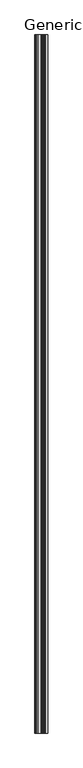
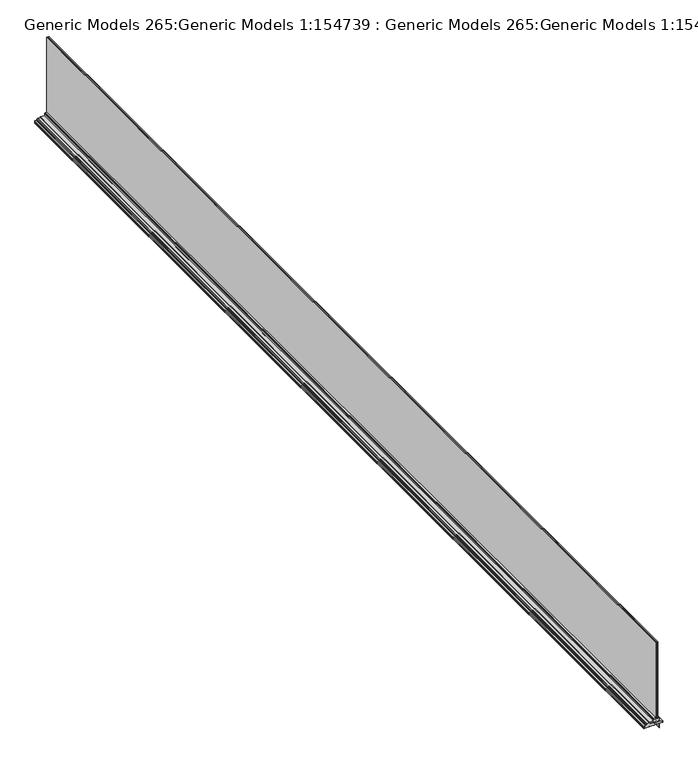
"""IFC4 building model written with IfcOpenShell, lengths in millimetres: proxy geometry, Generic Models 265:Generic Models 1:154739 : Generic Models 265:Generic Models 1:154739."""

from ifc_helpers import new_model, si_unit, point, frame, frame_2d, origin, place, context, project, spatial, polyline, circle_curve, trimmed, segment, composite_curve, outline, extrude, source, transform, mapped, element, save


def generic_models_265_generic_models_1_154739_generic_models_7b3244d4(model_context):
    return source(origin(), model_context, "Body", "SweptSolid", [
        extrude(outline(polyline([(1586.584463, 8383.5218843), (1586.584463, 496.8218843), (1581.821963, 496.8218843), (1581.821963, 8383.5218843), (1586.584463, 8383.5218843)])), frame((0.0, 0.0, 228.0707428), z_axis=(0.0, 0.0, 1.0), x_axis=(1.0, 0.0, 0.0)), (0.0, 0.0, 1.0), 602.3375481),
        extrude(outline(polyline([(1581.028213, 8383.5218843), (1581.028213, 496.8218843), (1574.679131, 496.8218843), (1574.679131, 8383.5218843), (1581.028213, 8383.5218843)])), frame((0.0, 0.0, 228.0707428), z_axis=(0.0, 0.0, 1.0), x_axis=(1.0, 0.0, 0.0)), (0.0, 0.0, 1.0), 6.35),
        extrude(outline(polyline([(1573.885381, 8383.5218843), (1573.885381, 496.8218843), (1569.122881, 496.8218843), (1569.122881, 8383.5218843), (1573.885381, 8383.5218843)])), frame((0.0, 0.0, 228.0707428), z_axis=(0.0, 0.0, 1.0), x_axis=(1.0, 0.0, 0.0)), (0.0, 0.0, 1.0), 602.3375481),
        extrude(outline(composite_curve([segment(polyline([(236.1161928, 1588.4013551), (231.8807536, 1588.4013551), (230.8576116, 1587.378213), (227.2769928, 1587.378213), (227.2769928, 1565.9408422), (229.6652816, 1568.329131), (239.5966816, 1568.329131), (238.5840316, 1556.5014505), (236.4216816, 1556.5014505), (236.4216816, 1552.733531), (228.8778816, 1552.733531), (228.8778816, 1554.333731), (227.2769928, 1554.333731), (227.2769928, 1552.453213), (208.9889928, 1552.453213)]), True, "CONTINUOUS"), segment(trimmed(circle_curve(frame_2d((208.9889928, 1553.266013)), 0.8128), [point((208.9889928, 1552.453213))], [point((208.1761928, 1553.266013))], False, "CARTESIAN"), True, "CONTINUOUS"), segment(polyline([(208.1761928, 1553.266013), (208.1761928, 1566.601013)]), True, "CONTINUOUS"), segment(trimmed(circle_curve(frame_2d((208.1761928, 1568.582213)), 1.9812), [point((208.1761928, 1566.601013))], [point((208.1761928, 1570.563413))], True, "CARTESIAN"), True, "CONTINUOUS"), segment(polyline([(208.1761928, 1570.563413), (208.1761928, 1582.755413), (202.8675928, 1582.755413), (202.8675928, 1588.368813), (210.7923928, 1588.368813), (210.7923928, 1590.273813), (207.4903928, 1590.273813), (207.4903928, 1591.950213), (205.4583928, 1591.950213), (205.4583928, 1594.515613)]), True, "CONTINUOUS"), segment(trimmed(circle_curve(frame_2d((207.8459928, 1594.515613)), 2.3876), [point((205.4583928, 1594.515613))], [point((207.8459928, 1596.903213))], False, "CARTESIAN"), True, "CONTINUOUS"), segment(polyline([(207.8459928, 1596.903213), (230.1471928, 1596.903213), (230.1471928, 1594.515613), (237.9530163, 1591.9802525), (238.1425666, 1589.537213), (236.1161928, 1589.537213), (236.1161928, 1588.4013551)]), True, "CONTINUOUS")], self_intersect=False)), frame((0.0, 496.8218843, 0.0), z_axis=(0.0, 1.0, 0.0), x_axis=(0.0, 0.0, 1.0)), (0.0, 0.0, 1.0), 7886.7),
        extrude(outline(composite_curve([segment(polyline([(190.97406, 1480.6982627), (183.0238428, 1480.6982627), (183.0238428, 1498.7668061), (186.1988428, 1498.7668061), (186.1988428, 1501.05281), (183.0238428, 1501.05281), (183.0238428, 1518.5605591), (186.1988428, 1518.5605591), (186.1988428, 1520.846563), (183.0238428, 1520.846563), (183.0238428, 1537.8736627), (185.1066428, 1537.8736627), (185.1066428, 1541.0486627), (183.0238428, 1541.0486627), (183.0238428, 1558.1480452), (186.1988428, 1558.1480452), (186.1988428, 1560.4340452), (183.0238428, 1560.4340452), (183.0238428, 1596.903213), (147.6519552, 1596.903213)]), True, "CONTINUOUS"), segment(trimmed(circle_curve(frame_2d((147.6542961, 1597.6017132)), 0.6985041), [point((147.6519552, 1596.903213))], [point((147.6567558, 1598.300213))], False, "CARTESIAN"), True, "CONTINUOUS"), segment(polyline([(147.6567558, 1598.300213), (183.0238428, 1598.300213), (183.0238428, 1623.1880474), (184.4208428, 1623.1880474), (184.4208428, 1616.8380474), (186.7068428, 1616.8380474), (186.7068428, 1624.741613), (195.6382661, 1624.741613), (198.060636, 1596.877813), (198.060636, 1561.927413), (202.9374286, 1561.927413), (202.9374286, 1557.9142859), (196.5184891, 1557.9142859), (196.5184891, 1555.9330115), (204.4686821, 1555.9330115), (204.4686821, 1547.5256758), (205.4084786, 1547.5256758), (205.4084786, 1529.9996758), (207.6944786, 1529.9996758), (207.6944786, 1547.5256758), (216.3812786, 1547.5256758), (216.3812786, 1550.5736487), (219.5562786, 1550.5736487), (219.5562786, 1521.1604247), (213.2244461, 1521.1604247), (213.2244461, 1502.1104247), (210.8368496, 1502.1104247), (210.8368496, 1500.5102316), (207.6618496, 1496.5732627), (207.6618496, 1494.9730696), (203.6994461, 1494.9730696), (203.6994461, 1491.7980696), (202.8866566, 1491.0106177), (202.8866566, 1480.6982627), (192.9552376, 1480.6982627), (192.9552376, 1488.6484557), (190.97406, 1488.6484557), (190.97406, 1480.6982627)]), True, "CONTINUOUS")], self_intersect=False)), frame((0.0, 496.8218843, 0.0), z_axis=(0.0, 1.0, 0.0), x_axis=(0.0, 0.0, 1.0)), (0.0, 0.0, 1.0), 7886.7),
    ])


if __name__ == "__main__":
    model = new_model("IFC4")
    model_context = context("Model", 3, world=origin())
    ifc_project = project(units=[si_unit("LENGTHUNIT", "METRE", prefix="MILLI")], contexts=[model_context])
    site = spatial("IfcSite", under=ifc_project)
    building = spatial("IfcBuilding", under=site)
    placement = place(None, origin())
    generic_models_265_generic_models_1_154739_generic_models_shape = generic_models_265_generic_models_1_154739_generic_models_7b3244d4(model_context)
    element("IfcBuildingElementProxy", 1, Name="Generic Models 265:Generic Models 1:154739 : Generic Models 265:Generic Models 1:154739", ObjectType="Generic Models 265:Generic Models 1:154739 : Generic Models 265:Generic Models 1:154739", at=placement, inside=building, context=model_context, shape_type="MappedRepresentation", body=[
        mapped(generic_models_265_generic_models_1_154739_generic_models_shape, transform((0.0, 0.0, 0.0), x_axis=(1.0, 0.0, 0.0), y_axis=(0.0, 1.0, 0.0), z_axis=(0.0, 0.0, 1.0))),
    ])
    save(model, "model.ifc")

# Revit data of these elements
# Type "Generic Models 265:Generic Models 1:154739 : Generic Models 265:Generic Models 1:154739"
#   NameOverride = "Generic Models 265:Generic Models 1:154739"
#   ObjectTypeOverride = "Generic Models 265:Generic Models 1"
#   Reference = "Generic Models 1"
#   Category = "Generic Models"
#   Tag = "154739"
# Element 1 (IfcBuildingElementProxy, "Generic Models 265:Generic Models 1:154739 : Generic Models 265:Generic Models 1:154739")
#   Materials on its faces: "_WINDOW PER SCHEDULE 24593"
# Materials
#   "_WINDOW PER SCHEDULE 24593": class "Unassigned", colour RGB 255 255 255, transparency 0
